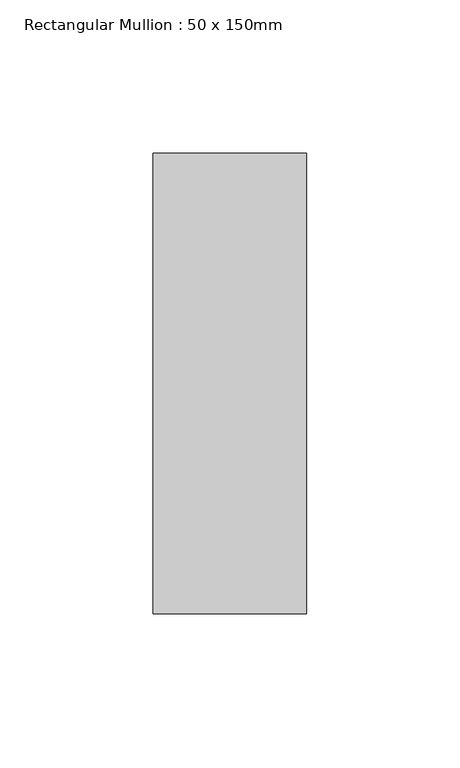
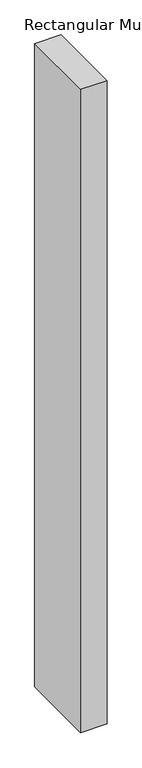
"""IFC4 building model written with IfcOpenShell, lengths in millimetres: member geometry, Rectangular Mullion : 50 x 150mm."""

from ifc_helpers import new_model, si_unit, frame, origin, place, context, project, spatial, polyline, outline, extrude, source, transform, mapped, element, save


def rectangular_mullion_50_x_150mm_87298841(model_context):
    return source(origin(), model_context, "Body", "SweptSolid", [
        extrude(outline(polyline([(0.0, 75.0), (0.0, -75.0), (-50.0, -75.0), (-50.0, 75.0), (0.0, 75.0)])), frame((0.0, 0.0, -1283.3333333), z_axis=(0.0, 0.0, 1.0), x_axis=(1.0, 0.0, 0.0)), (0.0, 0.0, 1.0), 1283.3333333),
    ])


if __name__ == "__main__":
    model = new_model("IFC4")
    model_context = context("Model", 3, world=origin())
    ifc_project = project(units=[si_unit("LENGTHUNIT", "METRE", prefix="MILLI")], contexts=[model_context])
    site = spatial("IfcSite", under=ifc_project)
    building = spatial("IfcBuilding", under=site)
    placement = place(None, origin())
    rectangular_mullion_50_x_150mm_shape = rectangular_mullion_50_x_150mm_87298841(model_context)
    element("IfcMember", 1, ObjectType="Rectangular Mullion : 50 x 150mm", at=placement, inside=building, context=model_context, shape_type="MappedRepresentation", body=[
        mapped(rectangular_mullion_50_x_150mm_shape, transform((0.0, 0.0, 0.0), x_axis=(1.0, 0.0, 0.0), y_axis=(0.0, 1.0, 0.0), z_axis=(0.0, 0.0, 1.0))),
    ])
    save(model, "model.ifc")

# Revit data of these elements
# Type "Rectangular Mullion : 50 x 150mm"
#   built-in parameter 1007304 = 0.492126 (stored number, unit not read)
#   built-in parameter 1007301 = 0.082021 (stored number, unit not read)
#   built-in parameter 1007300 = 0.082021 (stored number, unit not read)
# Element 1 (IfcMember, "Rectangular Mullion : 50 x 150mm")
#   Materials on its faces: "Metal - Aluminium"
# Materials
#   "Metal - Aluminium": class "Metal", colour RGB 247 247 247, transparency 0
